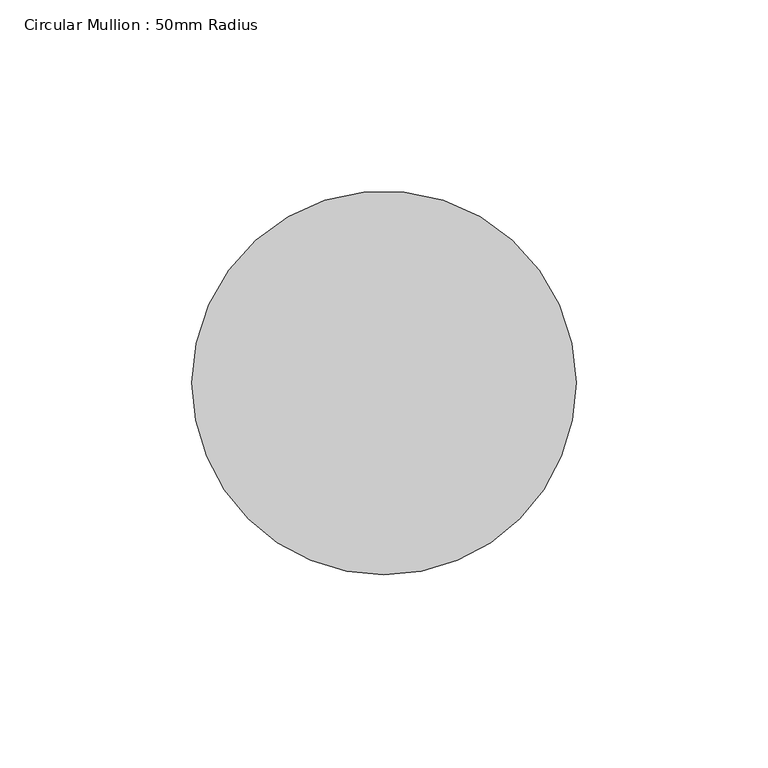
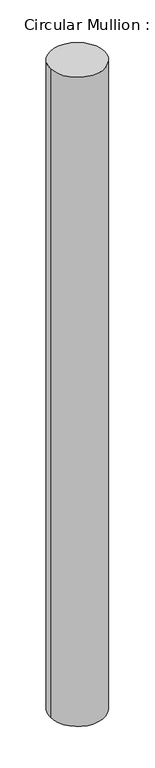
"""IFC4 building model written with IfcOpenShell, lengths in millimetres: member geometry, Circular Mullion : 50mm Radius."""

import ifcopenshell
import ifcopenshell.guid

model = None  # the IFC model being written
_history = None  # IfcOwnerHistory: only IFC2X3 demands one
_inside = {}  # id of a spatial element -> (the spatial element, [elements in it])
_under = {}  # id of a project, library or spatial element -> (it, [spatial elements below it])
_declared = {}  # id of a project -> (the project, [libraries it declares])
_typed = {}  # id of a type object -> (the type object, [elements of that type])
_made_of = {}  # id of a material, layer set ... -> (it, [elements and type objects made of it])


def new_model(schema):
    """Start an empty IFC model of exactly this schema.

    Asked for "IFC4X3", IfcOpenShell would pick the latest addendum, in which some entities
    have other attributes; the version numbers below select the first issue.
    IFC2X3 requires an IfcOwnerHistory on every rooted entity: one is made here for all.
    """
    global model, _history
    if schema == "IFC4X3":
        model = ifcopenshell.file(schema_version=(4, 3, 0, 0))
    else:
        model = ifcopenshell.file(schema=schema)
    _inside.clear()
    _under.clear()
    _declared.clear()
    _typed.clear()
    _made_of.clear()
    _history = None
    if model.schema == "IFC2X3":
        org = make("IfcOrganization", Name="unknown")
        user = make(
            "IfcPersonAndOrganization",
            ThePerson=make("IfcPerson", FamilyName="unknown"),
            TheOrganization=org,
        )
        app = make(
            "IfcApplication",
            ApplicationDeveloper=org,
            Version="unknown",
            ApplicationFullName="unknown",
            ApplicationIdentifier="unknown",
        )
        _history = make(
            "IfcOwnerHistory",
            OwningUser=user,
            OwningApplication=app,
            ChangeAction="ADDED",
            CreationDate=0,
        )
    return model


def make(cls, **values):
    """One entity of the class cls with the attributes given. An attribute that is None is left unset."""
    return model.create_entity(
        cls, **{name: value for name, value in values.items() if value is not None}
    )


def rooted(cls, **values):
    """An entity with a GlobalId (a new one), such as an element, a storey or a relation."""
    return make(cls, GlobalId=ifcopenshell.guid.new(), OwnerHistory=_history, **values)


def si_unit(unit_type, name, prefix=None):
    """IfcSIUnit, for example si_unit("LENGTHUNIT", "METRE", prefix="MILLI")."""
    return make("IfcSIUnit", UnitType=unit_type, Prefix=prefix, Name=name)


def assignment(units):
    """IfcUnitAssignment: the units of a project."""
    return None if units is None else make("IfcUnitAssignment", Units=units)


def point(xyz):
    """IfcCartesianPoint."""
    return None if xyz is None else make("IfcCartesianPoint", Coordinates=xyz)


def direction(xyz):
    """IfcDirection."""
    return None if xyz is None else make("IfcDirection", DirectionRatios=xyz)


def frame(location, z_axis=None, x_axis=None):
    """IfcAxis2Placement3D, a coordinate frame: its origin and axes. An axis left out is left unset."""
    return make(
        "IfcAxis2Placement3D",
        Location=point(location),
        Axis=direction(z_axis),
        RefDirection=direction(x_axis),
    )


def origin():
    """The frame at (0, 0, 0) with its axes left unset."""
    return frame((0.0, 0.0, 0.0))


def place(relative_to, where):
    """IfcLocalPlacement: puts the frame where relative to a parent placement (None: the world)."""
    return make(
        "IfcLocalPlacement", PlacementRelTo=relative_to, RelativePlacement=where
    )


def context(
    kind, dimensions, precision=None, world=None, true_north=None, identifier=None
):
    """IfcGeometricRepresentationContext, for example the 3D "Model" context."""
    return make(
        "IfcGeometricRepresentationContext",
        ContextIdentifier=identifier,
        ContextType=kind,
        CoordinateSpaceDimension=dimensions,
        Precision=precision,
        WorldCoordinateSystem=world,
        TrueNorth=true_north,
    )


def project(units=None, contexts=None):
    """IfcProject with its units and contexts."""
    return rooted(
        "IfcProject",
        Name="project",
        RepresentationContexts=contexts,
        UnitsInContext=assignment(units),
    )


def spatial(cls, under=None, at=None, **own):
    """A site, building, storey or space (cls), placed at a placement, below another one or the project."""
    s = rooted(cls, ObjectPlacement=at, **own)
    if under is not None:
        _under.setdefault(under.id(), (under, []))[1].append(s)
    return s


def ellipse_curve(where, semi_axis1, semi_axis2):
    """IfcEllipse in the frame where."""
    return make(
        "IfcEllipse", Position=where, SemiAxis1=semi_axis1, SemiAxis2=semi_axis2
    )


def shape(context_of_items, identifier, shape_type, items):
    """IfcShapeRepresentation: the items that make up one representation, for example the "Body"."""
    return make(
        "IfcShapeRepresentation",
        ContextOfItems=context_of_items,
        RepresentationIdentifier=identifier,
        RepresentationType=shape_type,
        Items=items,
    )


def source(mapping_origin, context_of_items, identifier, shape_type, items):
    """IfcRepresentationMap: a shape defined once, which mapped items show again and again."""
    return make(
        "IfcRepresentationMap",
        MappingOrigin=mapping_origin,
        MappedRepresentation=shape(context_of_items, identifier, shape_type, items),
    )


def transform(
    local_origin,
    x_axis=None,
    y_axis=None,
    z_axis=None,
    scale=None,
    scale2=None,
    scale3=None,
    uniform=True,
):
    """IfcCartesianTransformationOperator3D, or its non-uniform kind. x_axis, y_axis, z_axis: its Axis1, 2, 3."""
    if uniform:
        return make(
            "IfcCartesianTransformationOperator3D",
            Axis1=direction(x_axis),
            Axis2=direction(y_axis),
            LocalOrigin=point(local_origin),
            Scale=scale,
            Axis3=direction(z_axis),
        )
    return make(
        "IfcCartesianTransformationOperator3DnonUniform",
        Axis1=direction(x_axis),
        Axis2=direction(y_axis),
        LocalOrigin=point(local_origin),
        Scale=scale,
        Axis3=direction(z_axis),
        Scale2=scale2,
        Scale3=scale3,
    )


def mapped(mapping_source, mapping_target):
    """IfcMappedItem: shows the shape of a source again, moved by a transform."""
    return make(
        "IfcMappedItem", MappingSource=mapping_source, MappingTarget=mapping_target
    )


def made_of(thing, what):
    """Note that an element or type object is made of a material, layer set ...; save() writes the relation."""
    if what is not None:
        _made_of.setdefault(what.id(), (what, []))[1].append(thing)
    return thing


def element(
    cls,
    number,
    at=None,
    inside=None,
    cuts=None,
    type_object=None,
    material=None,
    context=None,
    identifier="Body",
    shape_type=None,
    held_by="IfcProductDefinitionShape",
    body=None,
    shapes=None,
    **own,
):
    """One element of the class cls, such as IfcWall. Its Tag is "e" and its number.

    at: its placement. inside: the storey or other place that contains it. cuts: it is an
    opening in that element (IfcRelVoidsElement). A single representation is given by context,
    identifier, shape_type and body (its items); several are given by shapes. held_by: the class
    of the entity that holds the representations. save() writes the other relations.
    """
    e = rooted(cls, Tag="e%d" % number, ObjectPlacement=at, **own)
    if body is not None:
        shapes = [shape(context, identifier, shape_type, body)]
    if shapes is not None:
        e.Representation = make(held_by, Representations=shapes)
    if inside is not None:
        _inside.setdefault(inside.id(), (inside, []))[1].append(e)
    if cuts is not None:
        rooted(
            "IfcRelVoidsElement", RelatingBuildingElement=cuts, RelatedOpeningElement=e
        )
    if type_object is not None:
        _typed.setdefault(type_object.id(), (type_object, []))[1].append(e)
    return made_of(e, material)


def aggregate(whole, parts):
    """IfcRelAggregates: a whole, such as a stair, and the parts it consists of."""
    return rooted("IfcRelAggregates", RelatingObject=whole, RelatedObjects=parts)


def save(model, path):
    """Write the relations noted so far, then the file.

    IfcRelAggregates (storeys below a building ...), IfcRelContainedInSpatialStructure (elements
    in a storey), IfcRelDefinesByType, IfcRelAssociatesMaterial and IfcRelDeclares: one each for
    every whole, place, type object, material and project.
    """
    for whole, parts in _under.values():
        aggregate(whole, parts)
    for where, things in _inside.values():
        rooted(
            "IfcRelContainedInSpatialStructure",
            RelatedElements=things,
            RelatingStructure=where,
        )
    for kind, things in _typed.values():
        rooted("IfcRelDefinesByType", RelatedObjects=things, RelatingType=kind)
    for what, things in _made_of.values():
        rooted("IfcRelAssociatesMaterial", RelatedObjects=things, RelatingMaterial=what)
    for by, libraries in _declared.values():
        rooted("IfcRelDeclares", RelatingContext=by, RelatedDefinitions=libraries)
    model.write(path)


def plane_surface(at):
    """IfcPlane: the flat surface through the origin of the frame at, square to its z axis."""
    return make("IfcPlane", Position=at)


def cylinder_surface(at, radius):
    """IfcCylindricalSurface: all points at the distance radius from the z axis of the frame at."""
    return make("IfcCylindricalSurface", Position=at, Radius=radius)


def advanced_brep(points, edges, surfaces, faces):
    """IfcAdvancedBrep: a solid bounded by faces that lie on surfaces and meet in shared edges.

    An edge is (start, end): straight between two places in points (the first is 0);
    or (start, end, curve); or (start, end, curve, False) where it runs against its curve.
    A face is (place in surfaces, loops), or (place, loops, False) where it looks against
    its surface's normal. A loop lists edges by number (the first is 1), with a minus sign
    where the edge is run from its end to its start. The first loop is the outer one.
    """
    corners = [point(p) for p in points]
    vertices = [make("IfcVertexPoint", VertexGeometry=c) for c in corners]
    made = []
    for start, end, *more in edges:
        made.append(
            make(
                "IfcEdgeCurve",
                EdgeStart=vertices[start],
                EdgeEnd=vertices[end],
                EdgeGeometry=more[0] if more else make("IfcPolyline", Points=[corners[start], corners[end]]),
                SameSense=more[1] if len(more) > 1 else True,
            )
        )
    hull = []
    for where, loops, *sense in faces:
        bounds = []
        for j, loop in enumerate(loops):
            ring = [make("IfcOrientedEdge", EdgeElement=made[abs(k) - 1], Orientation=k > 0) for k in loop]
            bounds.append(
                make(
                    "IfcFaceOuterBound" if j == 0 else "IfcFaceBound",
                    Bound=make("IfcEdgeLoop", EdgeList=ring),
                    Orientation=True,
                )
            )
        hull.append(make("IfcAdvancedFace", Bounds=bounds, FaceSurface=surfaces[where], SameSense=sense[0] if sense else True))
    return make("IfcAdvancedBrep", Outer=make("IfcClosedShell", CfsFaces=hull))


def circular_mullion_50mm_radius_bb41db6f(model_context):
    return source(origin(), model_context, "Body", "AdvancedBrep", [
        advanced_brep(
        [(-100.0, 0.0, 1.0641511), (0.0, 0.0, 0.0), (0.0, 0.0, -1259.8323479), (-100.0, 0.0, -1260.833319)],
        [
            (0, 1, ellipse_curve(frame((-50.0, 0.0, 0.5320756), z_axis=(-0.010639104733634393, -0.018413428254985806, -0.99977385198372), x_axis=(-0.5001727466316216, -0.8656644723201623, 0.02126605016533696)), 50.01131, 50.0)),
            (1, 2),
            (2, 3, ellipse_curve(frame((-50.0, 0.0, -1260.3328335), z_axis=(-0.010007708115976508, -0.017320650562617813, 0.9997999004012519), x_axis=(0.5001857782872434, 0.8656870266103899, 0.02000397854544681)), 50.010007, 50.0)),
            (3, 0),
            (1, 0, ellipse_curve(frame((-50.0, 0.0, 0.5320756), z_axis=(-0.010639104733634393, -0.018413428254985806, -0.99977385198372), x_axis=(-0.5001727466316216, -0.8656644723201623, 0.02126605016533696)), 50.01131, 50.0)),
            (3, 2, ellipse_curve(frame((-50.0, 0.0, -1260.3328335), z_axis=(-0.010007708115976508, -0.017320650562617813, 0.9997999004012519), x_axis=(0.5001857782872434, 0.8656870266103899, 0.02000397854544681)), 50.010007, 50.0)),
        ],
        [
            cylinder_surface(frame((-50.0, 0.0, 0.0), z_axis=(0.0, 0.0, 1.0), x_axis=(1.0, 0.0, 0.0)), 50.0),
            plane_surface(frame((-263.9142148, 152.4871378, 0.0), z_axis=(0.010639104733634393, 0.018413428254985806, 0.99977385198372), x_axis=(0.5001727466316203, 0.8656644723201631, -0.021266050165339855))),
            plane_surface(frame((-263.9142148, 152.4871378, -1259.8323479), z_axis=(0.010007708115976508, 0.017320650562617813, -0.9997999004012519), x_axis=(0.5001857782872433, 0.8656870266103899, 0.020003978545451773))),
        ],
        [
            (0, [[1, 2, 3, 4]]),
            (0, [[5, -4, 6, -2]]),
            (1, [[-1, -5]]),
            (2, [[-6, -3]]),
        ],
    ),
    ])


if __name__ == "__main__":
    model = new_model("IFC4")
    model_context = context("Model", 3, world=origin())
    ifc_project = project(units=[si_unit("LENGTHUNIT", "METRE", prefix="MILLI")], contexts=[model_context])
    site = spatial("IfcSite", under=ifc_project)
    building = spatial("IfcBuilding", under=site)
    placement = place(None, origin())
    circular_mullion_50mm_radius_shape = circular_mullion_50mm_radius_bb41db6f(model_context)
    element("IfcMember", 1, ObjectType="Circular Mullion : 50mm Radius", at=placement, inside=building, context=model_context, shape_type="MappedRepresentation", body=[
        mapped(circular_mullion_50mm_radius_shape, transform((0.0, 0.0, 0.0), x_axis=(1.0, 0.0, 0.0), y_axis=(0.0, 1.0, 0.0), z_axis=(0.0, 0.0, 1.0))),
    ])
    save(model, "model.ifc")

# Revit data of these elements
# Type "Circular Mullion : 50mm Radius"
#   built-in parameter 1007350 = 0.164042 (stored number, unit not read)
# Element 1 (IfcMember, "Circular Mullion : 50mm Radius")
#   Materials on its faces: "Aluminium"
# Materials
#   "Aluminium": class "Metal", colour RGB 247 247 247, transparency 0, Description = "Aluminium 6061", Cost = 0
